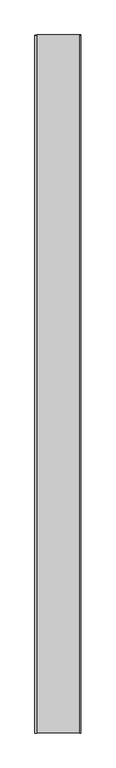
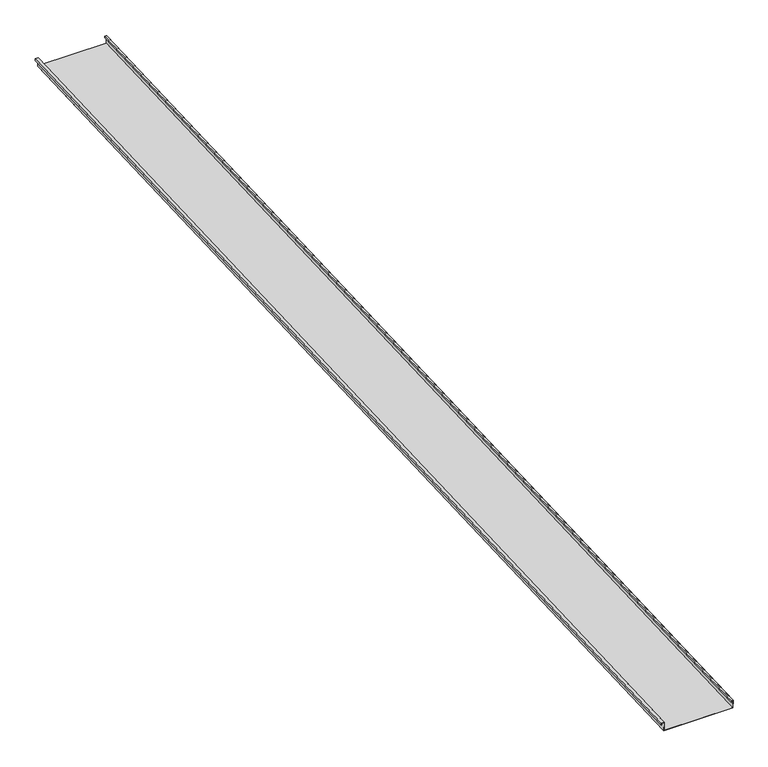
"""IFC4 building model written with IfcOpenShell, lengths in millimetres: proxy geometry, Generic Models 2:Generic Models 2:310765:Generic Models 2:310765 : Generic Models 2:Generic Models 2:310765:100 : Generic Models 2:Generic Models 2:310765:Generic Models 2:310765 : Generic Models 2:Generic Models 2:310765:300385."""

from ifc_helpers import new_model, si_unit, frame, origin, place, context, project, spatial, polyline, outline, extrude, source, transform, mapped, element, save


def generic_models_c4001488(model_context):
    return source(origin(), model_context, "Body", "SweptSolid", [
        extrude(outline(polyline([(1.5875, 0.0), (1.5875, 50.8), (407.9875, 50.8), (407.9875, 1.5875), (396.875, 1.5875), (396.875, 11.1125), (398.4625, 11.1125), (398.4625, 3.175), (406.4, 3.175), (406.4, 49.2125), (3.175, 49.2125), (3.175, -1.5874999), (-14.2875, -1.5874999), (-14.2875, 9.525), (-12.7, 9.525), (-12.7, 0.0), (1.5875, 0.0)])), frame((612327.9763073, -581354.4345603, 3902.6697972), z_axis=(0.0, 0.9991330730923568, 0.041630544712067834), x_axis=(1.0, 0.0, 0.0)), (0.0, 0.0, 1.0), 6400.8),
    ])


if __name__ == "__main__":
    model = new_model("IFC4")
    model_context = context("Model", 3, world=origin())
    ifc_project = project(units=[si_unit("LENGTHUNIT", "METRE", prefix="MILLI")], contexts=[model_context])
    site = spatial("IfcSite", under=ifc_project)
    building = spatial("IfcBuilding", under=site)
    placement = place(None, origin())
    generic_models_shape = generic_models_c4001488(model_context)
    element("IfcBuildingElementProxy", 1, Name="Generic Models 2:Generic Models 2:310765:Generic Models 2:310765 : Generic Models 2:Generic Models 2:310765:100 : Generic Models 2:Generic Models 2:310765:Generic Models 2:310765 : Generic Models 2:Generic Models 2:310765:300385", ObjectType="Generic Models 2:Generic Models 2:310765:Generic Models 2:310765 : Generic Models 2:Generic Models 2:310765:100 : Generic Models 2:Generic Models 2:310765:Generic Models 2:310765 : Generic Models 2:Generic Models 2:310765:300385", at=placement, inside=building, context=model_context, shape_type="MappedRepresentation", body=[
        mapped(generic_models_shape, transform((0.0, 0.0, 0.0), x_axis=(1.0, 0.0, 0.0), y_axis=(0.0, 1.0, 0.0), z_axis=(0.0, 0.0, 1.0))),
    ])
    save(model, "model.ifc")

# Revit data of these elements
# Type "Generic Models 2:Generic Models 2:310765:Generic Models 2:310765 : Generic Models 2:Generic Models 2:310765:100 : Generic Models 2:Generic Models 2:310765:Generic Models 2:310765 : Generic Models 2:Generic Models 2:310765:300385"
#   NameOverride = "Generic Models 2:Generic Models 2:310765:Generic Models 2:310765 : Generic Models 2:Generic Models 2:310765:300385"
#   ObjectTypeOverride = "Generic Models 2:310765 : Generic Models 2:Generic Models 2:310765"
#   Reference = "Generic Models 2"
#   Tag = "300385"
# Element 1 (IfcBuildingElementProxy, "Generic Models 2:Generic Models 2:310765:Generic Models 2:310765 : Generic Models 2:Generic Models 2:310765:100 : Generic Models 2:Generic Models 2:310765:Generic Models 2:310765 : Generic Models 2:Generic Models 2:310765:300385")
#   Materials on its faces: "THERMAL BROKEN ALUMINUM STOREFRONT FOR POLYCARBONATE"
# Materials
#   "THERMAL BROKEN ALUMINUM STOREFRONT FOR POLYCARBONATE": class "Unassigned", colour RGB 244 244 244, transparency 0, Keynote = "M07611300.01", Cost = 0
